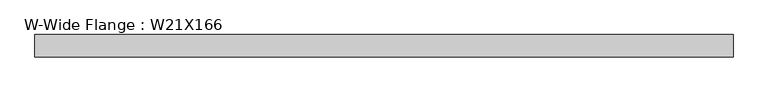
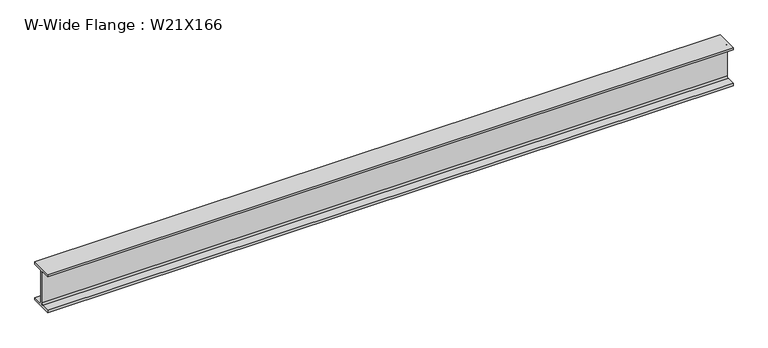
"""IFC4 building model written with IfcOpenShell, lengths in millimetres: beam geometry, W-Wide Flange : W21X166."""

from ifc_helpers import new_model, si_unit, point, frame, frame_2d, origin, place, context, project, spatial, polyline, circle_curve, trimmed, segment, composite_curve, outline, extrude, source, transform, mapped, element, save


def w_wide_flange_w21x166_c1e76bd8(model_context):
    return source(origin(), model_context, "Body", "SweptSolid", [
        extrude(outline(composite_curve([segment(polyline([(157.48, -251.206), (157.48, -285.75), (-157.48, -285.75), (-157.48, -251.206), (-32.131, -251.206)]), True, "CONTINUOUS"), segment(trimmed(circle_curve(frame_2d((-32.131, -228.6)), 22.606), [point((-32.131, -251.206))], [point((-9.525, -228.6))], True, "CARTESIAN"), True, "CONTINUOUS"), segment(polyline([(-9.525, -228.6), (-9.525, 228.6)]), True, "CONTINUOUS"), segment(trimmed(circle_curve(frame_2d((-32.131, 228.6)), 22.606), [point((-9.525, 228.6))], [point((-32.131, 251.206))], True, "CARTESIAN"), True, "CONTINUOUS"), segment(polyline([(-32.131, 251.206), (-157.48, 251.206), (-157.48, 285.75), (157.48, 285.75), (157.48, 251.206), (32.131, 251.206)]), True, "CONTINUOUS"), segment(trimmed(circle_curve(frame_2d((32.131, 228.6)), 22.606), [point((32.131, 251.206))], [point((9.525, 228.6))], True, "CARTESIAN"), True, "CONTINUOUS"), segment(polyline([(9.525, 228.6), (9.525, -228.6)]), True, "CONTINUOUS"), segment(trimmed(circle_curve(frame_2d((32.131, -228.6)), 22.606), [point((9.525, -228.6))], [point((32.131, -251.206))], True, "CARTESIAN"), True, "CONTINUOUS"), segment(polyline([(32.131, -251.206), (157.48, -251.206)]), True, "CONTINUOUS")], self_intersect=False)), frame((-4963.0833359, 0.0, 0.0), z_axis=(1.0, 0.0, 0.0), x_axis=(0.0, 1.0, 0.0)), (0.0, 0.0, 1.0), 9743.826275),
    ])


if __name__ == "__main__":
    model = new_model("IFC4")
    model_context = context("Model", 3, world=origin())
    ifc_project = project(units=[si_unit("LENGTHUNIT", "METRE", prefix="MILLI")], contexts=[model_context])
    site = spatial("IfcSite", under=ifc_project)
    building = spatial("IfcBuilding", under=site)
    placement = place(None, origin())
    w_wide_flange_w21x166_shape = w_wide_flange_w21x166_c1e76bd8(model_context)
    element("IfcBeam", 1, ObjectType="W-Wide Flange : W21X166", at=placement, inside=building, context=model_context, shape_type="MappedRepresentation", body=[
        mapped(w_wide_flange_w21x166_shape, transform((0.0, 0.0, 0.0), x_axis=(1.0, 0.0, 0.0), y_axis=(0.0, 1.0, 0.0), z_axis=(0.0, 0.0, 1.0))),
    ])
    save(model, "model.ifc")

# Revit data of these elements
# Type "W-Wide Flange : W21X166"
#   Assembly Code = "B10"
#   W = 166
#   Length [instance default] = 5' - 0"
#   bf = 1' - 0.4"
#   d = 1' - 10 1/2"
#   k = 0' - 2 1/4"
#   k2 = 0' - 0.89"
#   tf = 0' - 1.36"
#   tw = 0' - 0 3/4"
#   A = 0.338889 SF
#   Structural Material [instance default] = Steel ASTM A992
# Element 1 (IfcBeam, "W-Wide Flange : W21X166")
#   Materials on its faces: "Steel ASTM A992"
# Materials
#   "Steel ASTM A992": class "Metal", colour RGB 199 199 199, transparency 0, Description = "Structural steel 50ksi", Cost = 0
